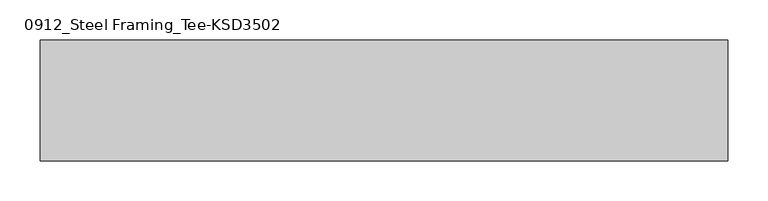
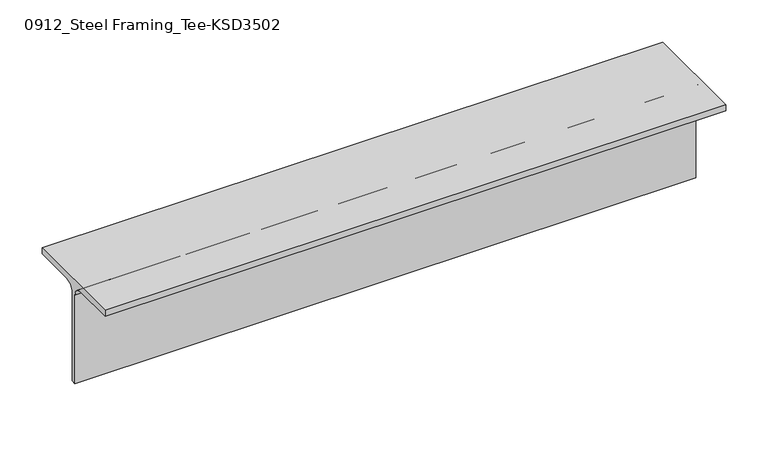
"""IFC4 building model written with IfcOpenShell, lengths in millimetres: member geometry, 0912_Steel Framing_Tee-KSD3502 : H_SB_ASB_CT-150x150x6.5x9."""

from ifc_helpers import new_model, si_unit, point, frame, frame_2d, origin, place, context, project, spatial, polyline, circle_curve, trimmed, segment, composite_curve, outline, extrude, source, transform, mapped, element, save


def member_0912_steel_framing_tee_ksd3502_6a8cd83b(model_context):
    return source(origin(), model_context, "Body", "SweptSolid", [
        extrude(outline(composite_curve([segment(polyline([(75.0, 75.0), (75.0, 66.0), (16.25, 66.0)]), True, "CONTINUOUS"), segment(trimmed(circle_curve(frame_2d((16.25, 53.0)), 13.0), [point((16.25, 66.0))], [point((3.25, 53.0))], True, "CARTESIAN"), True, "CONTINUOUS"), segment(polyline([(3.25, 53.0), (3.25, -75.0), (-3.25, -75.0), (-3.25, 53.0)]), True, "CONTINUOUS"), segment(trimmed(circle_curve(frame_2d((-16.25, 53.0)), 13.0), [point((-3.25, 53.0))], [point((-16.25, 66.0))], True, "CARTESIAN"), True, "CONTINUOUS"), segment(polyline([(-16.25, 66.0), (-75.0, 66.0), (-75.0, 75.0), (75.0, 75.0)]), True, "CONTINUOUS")], self_intersect=False)), frame((-353.0, 0.0, 0.0), z_axis=(1.0, 0.0, 0.0), x_axis=(0.0, 1.0, 0.0)), (0.0, 0.0, 1.0), 853.0),
    ])


if __name__ == "__main__":
    model = new_model("IFC4")
    model_context = context("Model", 3, world=origin())
    ifc_project = project(units=[si_unit("LENGTHUNIT", "METRE", prefix="MILLI")], contexts=[model_context])
    site = spatial("IfcSite", under=ifc_project)
    building = spatial("IfcBuilding", under=site)
    placement = place(None, origin())
    member_0912_steel_framing_tee_ksd3502_shape = member_0912_steel_framing_tee_ksd3502_6a8cd83b(model_context)
    element("IfcMember", 1, ObjectType="0912_Steel Framing_Tee-KSD3502 : H_SB_ASB_CT-150x150x6.5x9", at=placement, inside=building, context=model_context, shape_type="MappedRepresentation", body=[
        mapped(member_0912_steel_framing_tee_ksd3502_shape, transform((0.0, 0.0, 0.0), x_axis=(1.0, 0.0, 0.0), y_axis=(0.0, 1.0, 0.0), z_axis=(0.0, 0.0, 1.0))),
    ])
    save(model, "model.ifc")

# Revit data of these elements
# Type "0912_Steel Framing_Tee-KSD3502 : H_SB_ASB_CT-150x150x6.5x9"
#   H_WM Code_1 = "S01AA003-00001 | Main Steel Structure Fabrication Work | Shelter/Building | Light Steel - Standard (30KG/M>Weight) | Material: (   )"
#   H_WM Code_2 = "S03AA029-00001 | Main Steel Structure Erection Work | Shelter/Building | Light Steel (30KG/M>Weight) | Material: (   )"
#   H_WM Code_3 = "S01AA010-00001 | Main Steel Structure Fabrication Work | Shelter/Building | Steel Painting/Coating | for Non-Fireproofed Steel Surface, Surface Preparation, Primer, Second & Final Coat | Material: (   )"
#   H_Q'ty Cal Type Tag = "SB-Q2"
#   Width = 15.0 cm
#   Web Thickness = 0.65 cm
#   Web Fillet = 1.3 cm
#   Section Area = 23.39 cm²
#   Perimeter = 0.60 m²/m
#   Nominal Weight = 18.40 kgf/m
#   Height = 15.0 cm
#   Flange Thickness = 0.9 cm
#   Centroid Vertical = 7.5 cm
#   Centroid Horizontal = 7.5 cm
#   Length [instance default] = 1.5000 m
#   Structural Material [instance default] = Steel, 45-345
#   Warping Constant = (empty or 0)
#   Torsional Moment of Inertia = 0
#   Section Name Key = ""
#   Plastic Modulus weak axis = 0
#   Plastic Modulus strong axis = 0
#   Moment of Inertia weak axis = 0
#   Moment of Inertia strong axis = 0
#   Elastic Modulus weak axis = 0
#   Elastic Modulus strong axis = 0
#   Bolt Spacing = 0
#   Assembly Code = ""
# Element 1 (IfcMember, "0912_Steel Framing_Tee-KSD3502 : H_SB_ASB_CT-150x150x6.5x9")
#   Structural Material = none
# Materials
#   "Steel, 45-345": class "Metal", colour RGB 189 187 185, transparency 0, Description = "Steel 345 MPa", Cost = 0
